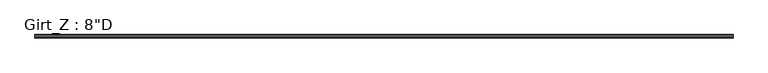
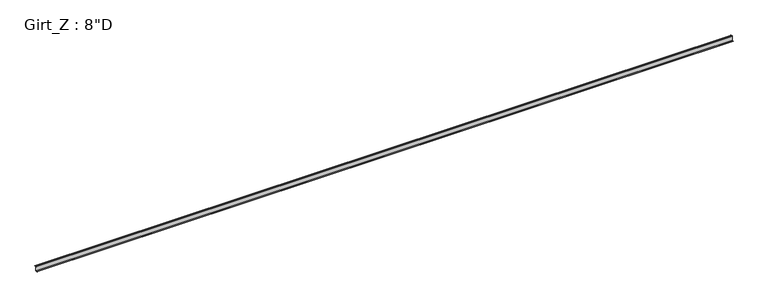
"""IFC4 building model written with IfcOpenShell, lengths in millimetres: beam geometry."""

from ifc_helpers import new_model, si_unit, point, frame, frame_2d, origin, place, context, project, spatial, polyline, circle_curve, trimmed, segment, composite_curve, outline, extrude, source, transform, mapped, element, save


def beam_533b4b39(model_context):
    return source(origin(), model_context, "Body", "SweptSolid", [
        extrude(outline(composite_curve([segment(polyline([(63.5, 101.6), (75.745104, 87.0068534), (73.6169367, 85.221109), (62.204539, 98.821875), (3.3005807, 98.821875)]), True, "CONTINUOUS"), segment(trimmed(circle_curve(frame_2d((3.3741066, 96.8381931)), 1.9850441), [point((3.3005807, 98.821875))], [point((1.3890625, 96.8381931))], True, "CARTESIAN"), True, "CONTINUOUS"), segment(polyline([(1.3890625, 96.8381931), (1.3890625, -96.8375)]), True, "CONTINUOUS"), segment(trimmed(circle_curve(frame_2d((-3.3734375, -96.8375)), 4.7625), [point((1.3890625, -96.8375))], [point((-3.3734375, -101.6))], False, "CARTESIAN"), True, "CONTINUOUS"), segment(polyline([(-3.3734375, -101.6), (-63.5, -101.6), (-75.745104, -87.0068534), (-73.6169367, -85.221109), (-62.204539, -98.821875), (-3.2694106, -98.821875)]), True, "CONTINUOUS"), segment(trimmed(circle_curve(frame_2d((-3.3748024, -96.8389339)), 1.9857399), [point((-3.2694106, -98.821875))], [point((-1.3890625, -96.8389339))], True, "CARTESIAN"), True, "CONTINUOUS"), segment(polyline([(-1.3890625, -96.8389339), (-1.3890625, 96.8375)]), True, "CONTINUOUS"), segment(trimmed(circle_curve(frame_2d((3.3734375, 96.8375)), 4.7625), [point((-1.3890625, 96.8375))], [point((3.3734375, 101.6))], False, "CARTESIAN"), True, "CONTINUOUS"), segment(polyline([(3.3734375, 101.6), (63.5, 101.6)]), True, "CONTINUOUS")], self_intersect=False)), frame((-15623.38125, 0.0, 0.0), z_axis=(1.0, 0.0, 0.0), x_axis=(0.0, 1.0, 0.0)), (0.0, 0.0, 1.0), 29895.5150467),
    ])


if __name__ == "__main__":
    model = new_model("IFC4")
    model_context = context("Model", 3, world=origin())
    ifc_project = project(units=[si_unit("LENGTHUNIT", "METRE", prefix="MILLI")], contexts=[model_context])
    site = spatial("IfcSite", under=ifc_project)
    building = spatial("IfcBuilding", under=site)
    placement = place(None, origin())
    beam_shape = beam_533b4b39(model_context)
    element("IfcBeam", 1, ObjectType="Girt_Z : 8\"D", at=placement, inside=building, context=model_context, shape_type="MappedRepresentation", body=[
        mapped(beam_shape, transform((0.0, 0.0, 0.0), x_axis=(1.0, 0.0, 0.0), y_axis=(0.0, 1.0, 0.0), z_axis=(0.0, 0.0, 1.0))),
    ])
    save(model, "model.ifc")

# Revit data of these elements
# Type "Girt_Z : 8\"D"
#   Web_Thickness = 0' - 0 7/64"
#   Length [instance default] = 10' - 0"
#   Leg_1 = 0' - 2 1/2"
#   Height = 0' - 8"
#   Structural Material [instance default] = none
# Element 1 (IfcBeam, "Girt_Z : 8\"D")
#   Structural Material = Steel
#   Materials on its faces: "Steel"
# Materials
#   "Steel": class "Metal", colour RGB 118 118 114, transparency 0, Description = "Steel, mill finish", Cost = 0
